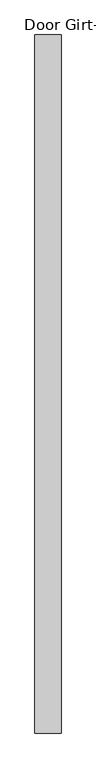
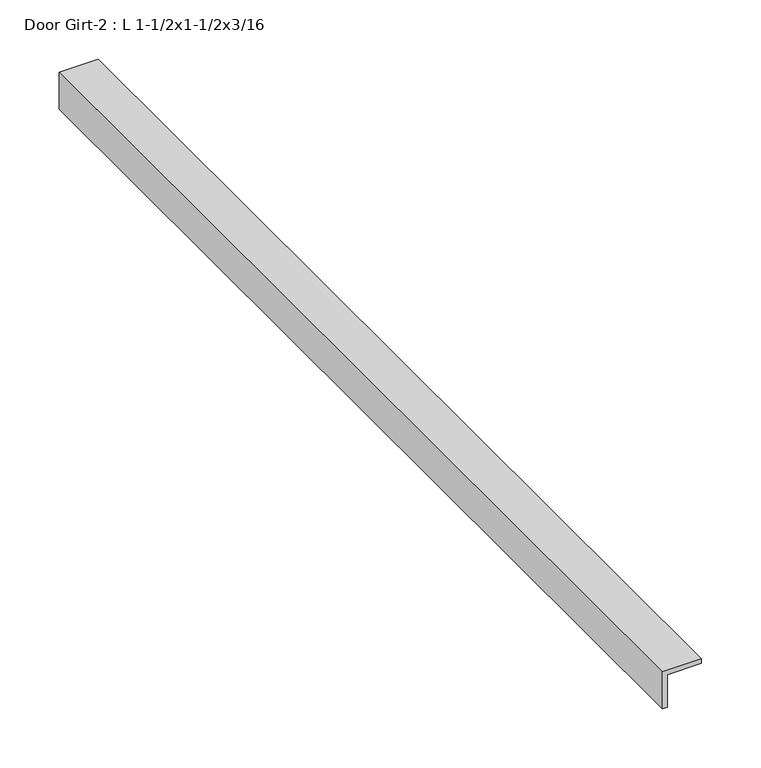
"""IFC4 building model written with IfcOpenShell, lengths in millimetres: proxy geometry, Door Girt-2 : L 1-1/2x1-1/2x3/16."""

from ifc_helpers import new_model, si_unit, frame, origin, place, context, project, spatial, polyline, outline, extrude, source, transform, mapped, element, save


def door_girt_2_l_1_1_2x1_1_2x3_16_599efec9(model_context):
    return source(origin(), model_context, "Body", "SweptSolid", [
        extrude(outline(polyline([(812.8, 587403.9934739), (812.8, 587365.8934739), (774.7, 587365.8934739), (774.7, 587370.6559739), (808.0375, 587370.6559739), (808.0375, 587403.9934739), (812.8, 587403.9934739)])), frame((0.0, -532839.3663841, 0.0), z_axis=(0.0, 1.0, 0.0), x_axis=(0.0, 0.0, 1.0)), (0.0, 0.0, 1.0), 1017.5875),
    ])


if __name__ == "__main__":
    model = new_model("IFC4")
    model_context = context("Model", 3, world=origin())
    ifc_project = project(units=[si_unit("LENGTHUNIT", "METRE", prefix="MILLI")], contexts=[model_context])
    site = spatial("IfcSite", under=ifc_project)
    building = spatial("IfcBuilding", under=site)
    placement = place(None, origin())
    door_girt_2_l_1_1_2x1_1_2x3_16_shape = door_girt_2_l_1_1_2x1_1_2x3_16_599efec9(model_context)
    element("IfcBuildingElementProxy", 1, Name="Door Girt-2 : L 1-1/2x1-1/2x3/16", ObjectType="Door Girt-2 : L 1-1/2x1-1/2x3/16", at=placement, inside=building, context=model_context, shape_type="MappedRepresentation", body=[
        mapped(door_girt_2_l_1_1_2x1_1_2x3_16_shape, transform((0.0, 0.0, 0.0), x_axis=(1.0, 0.0, 0.0), y_axis=(0.0, 1.0, 0.0), z_axis=(0.0, 0.0, 1.0))),
    ])
    save(model, "model.ifc")

# Revit data of these elements
# Element 1 (IfcBuildingElementProxy, "Door Girt-2 : L 1-1/2x1-1/2x3/16")
#   Materials on its faces: "1-1/2\"X1-1/2\" GALV. STL L"
# Materials
#   "1-1/2\"X1-1/2\" GALV. STL L": class "Generic", colour RGB 211 211 207, transparency 0, Cost = 0
